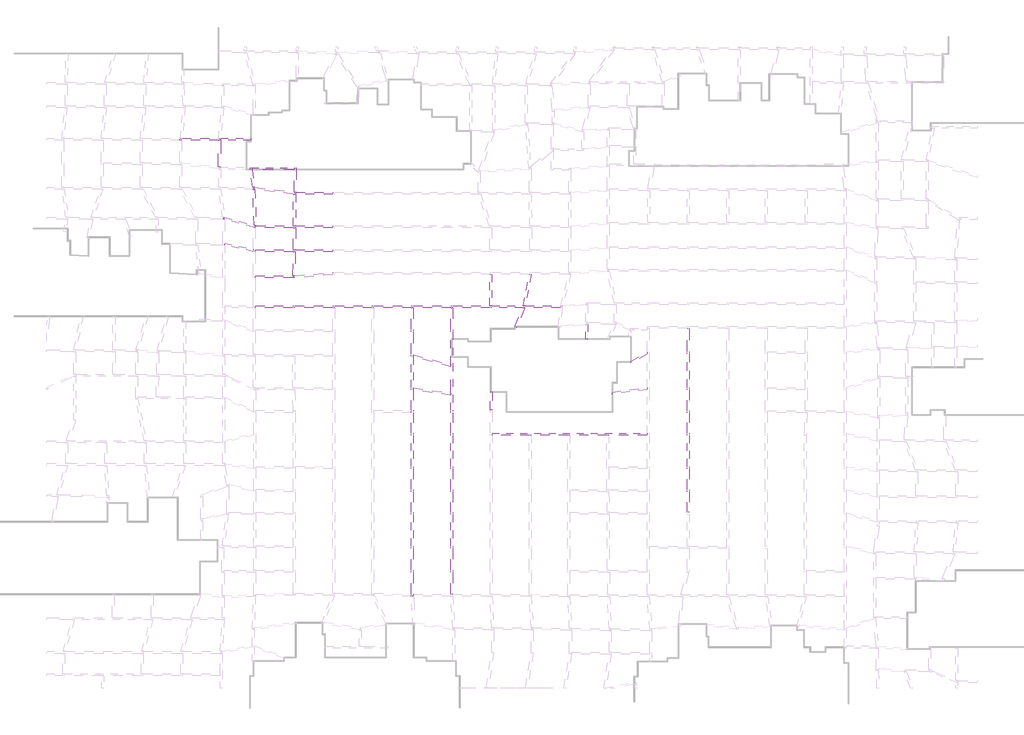
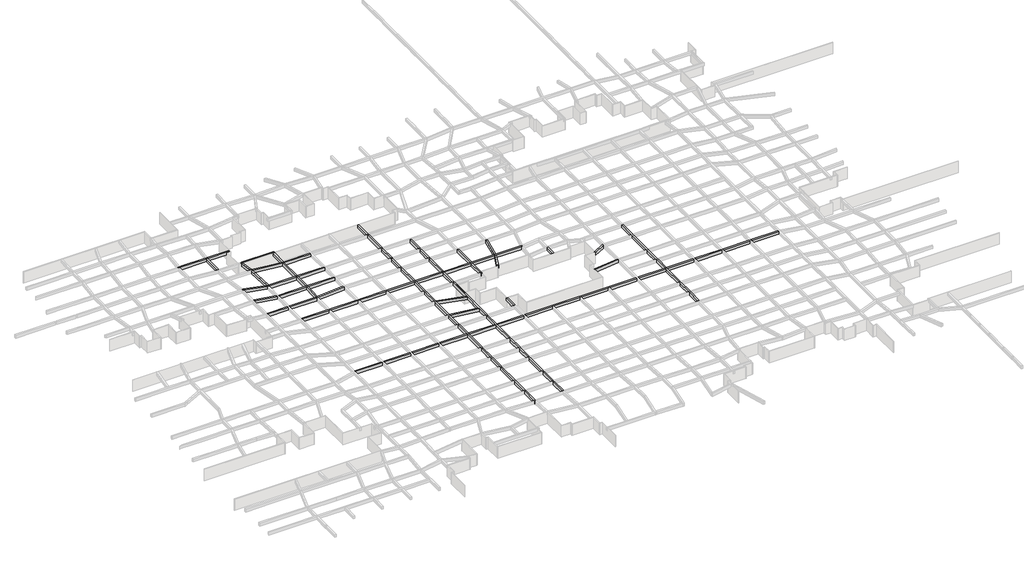
# One storey, part 28 of 45: 32 beams.
# Revit data of these elements (continued)
# Type "混凝土 - 矩形梁 : KL_beam"
#   Length [instance default] = 1524 mm
#   b = 400 mm
#   h = 800 mm
#   Structural Material [instance default] = 混凝土 - 现场浇注混凝土
#   Assembly Code = ""
# Elements 1, 2, 3, 4, 5, 6, 7, 8, 9, 10, 11, 12, 13, 14, 15, 16, 17, 18, 19, 20, 21, 22, 23, 24, 25, 26, 27, 28, 29, 30, 31, 32 (IfcBeam, "混凝土 - 矩形梁 : KL_beam")
#   Comments = ""
#   Structural Material = none
#   Phase Created = 新构造
# Materials
#   "混凝土 - 现场浇注混凝土": class "混凝土", colour RGB 192 192 192, transparency 0
